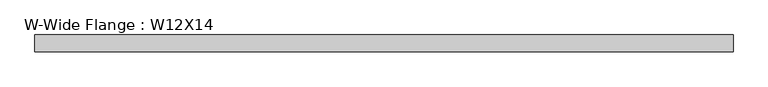
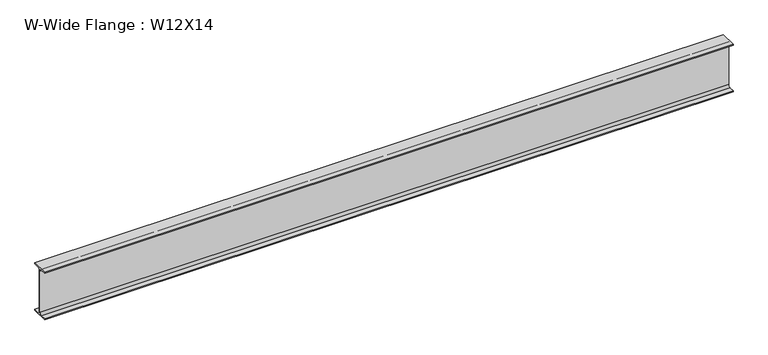
"""IFC4 building model written with IfcOpenShell, lengths in millimetres: beam geometry, W-Wide Flange : W12X14."""

import ifcopenshell
import ifcopenshell.guid

model = None  # the IFC model being written
_history = None  # IfcOwnerHistory: only IFC2X3 demands one
_inside = {}  # id of a spatial element -> (the spatial element, [elements in it])
_under = {}  # id of a project, library or spatial element -> (it, [spatial elements below it])
_declared = {}  # id of a project -> (the project, [libraries it declares])
_typed = {}  # id of a type object -> (the type object, [elements of that type])
_made_of = {}  # id of a material, layer set ... -> (it, [elements and type objects made of it])


def new_model(schema):
    """Start an empty IFC model of exactly this schema.

    Asked for "IFC4X3", IfcOpenShell would pick the latest addendum, in which some entities
    have other attributes; the version numbers below select the first issue.
    IFC2X3 requires an IfcOwnerHistory on every rooted entity: one is made here for all.
    """
    global model, _history
    if schema == "IFC4X3":
        model = ifcopenshell.file(schema_version=(4, 3, 0, 0))
    else:
        model = ifcopenshell.file(schema=schema)
    _inside.clear()
    _under.clear()
    _declared.clear()
    _typed.clear()
    _made_of.clear()
    _history = None
    if model.schema == "IFC2X3":
        org = make("IfcOrganization", Name="unknown")
        user = make(
            "IfcPersonAndOrganization",
            ThePerson=make("IfcPerson", FamilyName="unknown"),
            TheOrganization=org,
        )
        app = make(
            "IfcApplication",
            ApplicationDeveloper=org,
            Version="unknown",
            ApplicationFullName="unknown",
            ApplicationIdentifier="unknown",
        )
        _history = make(
            "IfcOwnerHistory",
            OwningUser=user,
            OwningApplication=app,
            ChangeAction="ADDED",
            CreationDate=0,
        )
    return model


def make(cls, **values):
    """One entity of the class cls with the attributes given. An attribute that is None is left unset."""
    return model.create_entity(
        cls, **{name: value for name, value in values.items() if value is not None}
    )


def rooted(cls, **values):
    """An entity with a GlobalId (a new one), such as an element, a storey or a relation."""
    return make(cls, GlobalId=ifcopenshell.guid.new(), OwnerHistory=_history, **values)


def si_unit(unit_type, name, prefix=None):
    """IfcSIUnit, for example si_unit("LENGTHUNIT", "METRE", prefix="MILLI")."""
    return make("IfcSIUnit", UnitType=unit_type, Prefix=prefix, Name=name)


def assignment(units):
    """IfcUnitAssignment: the units of a project."""
    return None if units is None else make("IfcUnitAssignment", Units=units)


def point(xyz):
    """IfcCartesianPoint."""
    return None if xyz is None else make("IfcCartesianPoint", Coordinates=xyz)


def direction(xyz):
    """IfcDirection."""
    return None if xyz is None else make("IfcDirection", DirectionRatios=xyz)


def frame(location, z_axis=None, x_axis=None):
    """IfcAxis2Placement3D, a coordinate frame: its origin and axes. An axis left out is left unset."""
    return make(
        "IfcAxis2Placement3D",
        Location=point(location),
        Axis=direction(z_axis),
        RefDirection=direction(x_axis),
    )


def frame_2d(location, x_axis=None):
    """IfcAxis2Placement2D, a coordinate frame in the plane: its origin and x axis."""
    return make(
        "IfcAxis2Placement2D", Location=point(location), RefDirection=direction(x_axis)
    )


def origin():
    """The frame at (0, 0, 0) with its axes left unset."""
    return frame((0.0, 0.0, 0.0))


def place(relative_to, where):
    """IfcLocalPlacement: puts the frame where relative to a parent placement (None: the world)."""
    return make(
        "IfcLocalPlacement", PlacementRelTo=relative_to, RelativePlacement=where
    )


def context(
    kind, dimensions, precision=None, world=None, true_north=None, identifier=None
):
    """IfcGeometricRepresentationContext, for example the 3D "Model" context."""
    return make(
        "IfcGeometricRepresentationContext",
        ContextIdentifier=identifier,
        ContextType=kind,
        CoordinateSpaceDimension=dimensions,
        Precision=precision,
        WorldCoordinateSystem=world,
        TrueNorth=true_north,
    )


def project(units=None, contexts=None):
    """IfcProject with its units and contexts."""
    return rooted(
        "IfcProject",
        Name="project",
        RepresentationContexts=contexts,
        UnitsInContext=assignment(units),
    )


def spatial(cls, under=None, at=None, **own):
    """A site, building, storey or space (cls), placed at a placement, below another one or the project."""
    s = rooted(cls, ObjectPlacement=at, **own)
    if under is not None:
        _under.setdefault(under.id(), (under, []))[1].append(s)
    return s


def polyline(points):
    """IfcPolyline through the points."""
    return make("IfcPolyline", Points=[point(p) for p in points])


def circle_curve(where, radius):
    """IfcCircle in the frame where."""
    return make("IfcCircle", Position=where, Radius=radius)


def trimmed(basis, trim1, trim2, sense, master):
    """IfcTrimmedCurve: the piece of a basis curve between two trims."""
    return make(
        "IfcTrimmedCurve",
        BasisCurve=basis,
        Trim1=trim1,
        Trim2=trim2,
        SenseAgreement=sense,
        MasterRepresentation=master,
    )


def segment(curve, same_sense, transition):
    """IfcCompositeCurveSegment."""
    return make(
        "IfcCompositeCurveSegment",
        Transition=transition,
        SameSense=same_sense,
        ParentCurve=curve,
    )


def composite_curve(segments, self_intersect=None):
    """IfcCompositeCurve: segments joined end to end."""
    return make("IfcCompositeCurve", Segments=segments, SelfIntersect=self_intersect)


def outline(outer, holes=None, kind="AREA"):
    """IfcArbitraryClosedProfileDef: a profile drawn as a closed curve; with holes, ...WithVoids."""
    if holes is None:
        return make("IfcArbitraryClosedProfileDef", ProfileType=kind, OuterCurve=outer)
    return make(
        "IfcArbitraryProfileDefWithVoids",
        ProfileType=kind,
        OuterCurve=outer,
        InnerCurves=holes,
    )


def extrude(swept, where, along, depth):
    """IfcExtrudedAreaSolid: the profile swept, set in the frame where, extruded along a direction by depth."""
    return make(
        "IfcExtrudedAreaSolid",
        SweptArea=swept,
        Position=where,
        ExtrudedDirection=direction(along),
        Depth=depth,
    )


def shape(context_of_items, identifier, shape_type, items):
    """IfcShapeRepresentation: the items that make up one representation, for example the "Body"."""
    return make(
        "IfcShapeRepresentation",
        ContextOfItems=context_of_items,
        RepresentationIdentifier=identifier,
        RepresentationType=shape_type,
        Items=items,
    )


def source(mapping_origin, context_of_items, identifier, shape_type, items):
    """IfcRepresentationMap: a shape defined once, which mapped items show again and again."""
    return make(
        "IfcRepresentationMap",
        MappingOrigin=mapping_origin,
        MappedRepresentation=shape(context_of_items, identifier, shape_type, items),
    )


def transform(
    local_origin,
    x_axis=None,
    y_axis=None,
    z_axis=None,
    scale=None,
    scale2=None,
    scale3=None,
    uniform=True,
):
    """IfcCartesianTransformationOperator3D, or its non-uniform kind. x_axis, y_axis, z_axis: its Axis1, 2, 3."""
    if uniform:
        return make(
            "IfcCartesianTransformationOperator3D",
            Axis1=direction(x_axis),
            Axis2=direction(y_axis),
            LocalOrigin=point(local_origin),
            Scale=scale,
            Axis3=direction(z_axis),
        )
    return make(
        "IfcCartesianTransformationOperator3DnonUniform",
        Axis1=direction(x_axis),
        Axis2=direction(y_axis),
        LocalOrigin=point(local_origin),
        Scale=scale,
        Axis3=direction(z_axis),
        Scale2=scale2,
        Scale3=scale3,
    )


def mapped(mapping_source, mapping_target):
    """IfcMappedItem: shows the shape of a source again, moved by a transform."""
    return make(
        "IfcMappedItem", MappingSource=mapping_source, MappingTarget=mapping_target
    )


def made_of(thing, what):
    """Note that an element or type object is made of a material, layer set ...; save() writes the relation."""
    if what is not None:
        _made_of.setdefault(what.id(), (what, []))[1].append(thing)
    return thing


def element(
    cls,
    number,
    at=None,
    inside=None,
    cuts=None,
    type_object=None,
    material=None,
    context=None,
    identifier="Body",
    shape_type=None,
    held_by="IfcProductDefinitionShape",
    body=None,
    shapes=None,
    **own,
):
    """One element of the class cls, such as IfcWall. Its Tag is "e" and its number.

    at: its placement. inside: the storey or other place that contains it. cuts: it is an
    opening in that element (IfcRelVoidsElement). A single representation is given by context,
    identifier, shape_type and body (its items); several are given by shapes. held_by: the class
    of the entity that holds the representations. save() writes the other relations.
    """
    e = rooted(cls, Tag="e%d" % number, ObjectPlacement=at, **own)
    if body is not None:
        shapes = [shape(context, identifier, shape_type, body)]
    if shapes is not None:
        e.Representation = make(held_by, Representations=shapes)
    if inside is not None:
        _inside.setdefault(inside.id(), (inside, []))[1].append(e)
    if cuts is not None:
        rooted(
            "IfcRelVoidsElement", RelatingBuildingElement=cuts, RelatedOpeningElement=e
        )
    if type_object is not None:
        _typed.setdefault(type_object.id(), (type_object, []))[1].append(e)
    return made_of(e, material)


def aggregate(whole, parts):
    """IfcRelAggregates: a whole, such as a stair, and the parts it consists of."""
    return rooted("IfcRelAggregates", RelatingObject=whole, RelatedObjects=parts)


def save(model, path):
    """Write the relations noted so far, then the file.

    IfcRelAggregates (storeys below a building ...), IfcRelContainedInSpatialStructure (elements
    in a storey), IfcRelDefinesByType, IfcRelAssociatesMaterial and IfcRelDeclares: one each for
    every whole, place, type object, material and project.
    """
    for whole, parts in _under.values():
        aggregate(whole, parts)
    for where, things in _inside.values():
        rooted(
            "IfcRelContainedInSpatialStructure",
            RelatedElements=things,
            RelatingStructure=where,
        )
    for kind, things in _typed.values():
        rooted("IfcRelDefinesByType", RelatedObjects=things, RelatingType=kind)
    for what, things in _made_of.values():
        rooted("IfcRelAssociatesMaterial", RelatedObjects=things, RelatingMaterial=what)
    for by, libraries in _declared.values():
        rooted("IfcRelDeclares", RelatingContext=by, RelatedDefinitions=libraries)
    model.write(path)


def w_wide_flange_w12x14_a768a83c(model_context):
    return source(origin(), model_context, "Body", "SweptSolid", [
        extrude(outline(composite_curve([segment(polyline([(50.419, -145.415), (50.419, -151.13), (-50.419, -151.13), (-50.419, -145.415), (-15.875, -145.415)]), True, "CONTINUOUS"), segment(trimmed(circle_curve(frame_2d((-15.875, -132.08)), 13.335), [point((-15.875, -145.415))], [point((-2.54, -132.08))], True, "CARTESIAN"), True, "CONTINUOUS"), segment(polyline([(-2.54, -132.08), (-2.54, 132.08)]), True, "CONTINUOUS"), segment(trimmed(circle_curve(frame_2d((-15.875, 132.08)), 13.335), [point((-2.54, 132.08))], [point((-15.875, 145.415))], True, "CARTESIAN"), True, "CONTINUOUS"), segment(polyline([(-15.875, 145.415), (-50.419, 145.415), (-50.419, 151.13), (50.419, 151.13), (50.419, 145.415), (15.875, 145.415)]), True, "CONTINUOUS"), segment(trimmed(circle_curve(frame_2d((15.875, 132.08)), 13.335), [point((15.875, 145.415))], [point((2.54, 132.08))], True, "CARTESIAN"), True, "CONTINUOUS"), segment(polyline([(2.54, 132.08), (2.54, -132.08)]), True, "CONTINUOUS"), segment(trimmed(circle_curve(frame_2d((15.875, -132.08)), 13.335), [point((2.54, -132.08))], [point((15.875, -145.415))], True, "CARTESIAN"), True, "CONTINUOUS"), segment(polyline([(15.875, -145.415), (50.419, -145.415)]), True, "CONTINUOUS")], self_intersect=False)), frame((-2082.8, 0.0, 0.0), z_axis=(1.0, 0.0, 0.0), x_axis=(0.0, 1.0, 0.0)), (0.0, 0.0, 1.0), 4165.6),
    ])


if __name__ == "__main__":
    model = new_model("IFC4")
    model_context = context("Model", 3, world=origin())
    ifc_project = project(units=[si_unit("LENGTHUNIT", "METRE", prefix="MILLI")], contexts=[model_context])
    site = spatial("IfcSite", under=ifc_project)
    building = spatial("IfcBuilding", under=site)
    placement = place(None, origin())
    w_wide_flange_w12x14_shape = w_wide_flange_w12x14_a768a83c(model_context)
    element("IfcBeam", 1, ObjectType="W-Wide Flange : W12X14", at=placement, inside=building, context=model_context, shape_type="MappedRepresentation", body=[
        mapped(w_wide_flange_w12x14_shape, transform((0.0, 0.0, 0.0), x_axis=(1.0, 0.0, 0.0), y_axis=(0.0, 1.0, 0.0), z_axis=(0.0, 0.0, 1.0))),
    ])
    save(model, "model.ifc")

# Revit data of these elements
# Type "W-Wide Flange : W12X14"
#   Assembly Code = "B10"
#   W = 14
#   Length [instance default] = 5' - 0"
#   bf = 0' - 3.97"
#   d = 0' - 11.9"
#   k = 0' - 0 3/4"
#   k2 = 0' - 0.525"
#   tf = 0' - 0.225"
#   tw = 0' - 0.2"
#   A = 0.0288889 SF
#   Structural Material [instance default] = Steel ASTM A992
# Element 1 (IfcBeam, "W-Wide Flange : W12X14")
#   Materials on its faces: "Steel ASTM A992"
# Materials
#   "Steel ASTM A992": class "Metal", colour RGB 199 199 199, transparency 0, Description = "Structural steel 50ksi", Cost = 0
